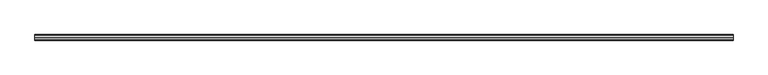
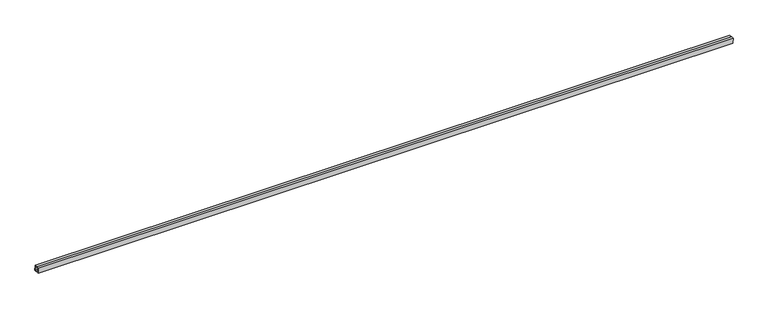
"""IFC4 building model written with IfcOpenShell, lengths in millimetres: proxy geometry, Inner panel:Inner panel:1:Inner panel:1 : Inner panel:Inner panel:300324:2:Inner panel:1:Inner panel:1 : Inner panel:Inner panel:300324:2 : Inner panel:Inner panel:1:Inner panel:1 : Inner panel:Inner panel:300324:300043:27 : Inner panel:Inner panel:1:Inner panel:1 : Inner panel:Inner panel:300324:2:Inner panel:1:Inner panel:1 : Inner panel:Inner panel:300324:2 : Inner panel:Inner panel:1:Inner panel:1 : Inner panel:Inner panel:300324:300043:308120."""

from ifc_helpers import new_model, si_unit, frame, origin, place, context, project, spatial, polyline, outline, extrude, source, transform, mapped, element, save


def generic_models_0cca4032(model_context):
    return source(origin(), model_context, "Body", "SweptSolid", [
        extrude(outline(polyline([(-567056.8153809, 8850.7720379), (-567038.5749577, 8851.5320556), (-567036.988834, 8813.4650855), (-567075.0558041, 8811.8789617), (-567076.6419278, 8849.9459318), (-567058.4015047, 8850.7059494), (-567058.3023719, 8848.3267638), (-567074.1636095, 8847.6658789), (-567072.7757512, 8814.3572801), (-567039.4671523, 8815.7451384), (-567040.8550106, 8849.0537372), (-567056.7162482, 8848.3928523), (-567056.8153809, 8850.7720379)])), frame((588245.3367242, 0.0, 0.0), z_axis=(1.0, 0.0, 0.0), x_axis=(0.0, 1.0, 0.0)), (0.0, 0.0, 1.0), 4876.8),
    ])


if __name__ == "__main__":
    model = new_model("IFC4")
    model_context = context("Model", 3, world=origin())
    ifc_project = project(units=[si_unit("LENGTHUNIT", "METRE", prefix="MILLI")], contexts=[model_context])
    site = spatial("IfcSite", under=ifc_project)
    building = spatial("IfcBuilding", under=site)
    placement = place(None, origin())
    generic_models_shape = generic_models_0cca4032(model_context)
    element("IfcBuildingElementProxy", 1, Name="Inner panel:Inner panel:1:Inner panel:1 : Inner panel:Inner panel:300324:2:Inner panel:1:Inner panel:1 : Inner panel:Inner panel:300324:2 : Inner panel:Inner panel:1:Inner panel:1 : Inner panel:Inner panel:300324:300043:27 : Inner panel:Inner panel:1:Inner panel:1 : Inner panel:Inner panel:300324:2:Inner panel:1:Inner panel:1 : Inner panel:Inner panel:300324:2 : Inner panel:Inner panel:1:Inner panel:1 : Inner panel:Inner panel:300324:300043:308120", ObjectType="Inner panel:Inner panel:1:Inner panel:1 : Inner panel:Inner panel:300324:2:Inner panel:1:Inner panel:1 : Inner panel:Inner panel:300324:2 : Inner panel:Inner panel:1:Inner panel:1 : Inner panel:Inner panel:300324:300043:27 : Inner panel:Inner panel:1:Inner panel:1 : Inner panel:Inner panel:300324:2:Inner panel:1:Inner panel:1 : Inner panel:Inner panel:300324:2 : Inner panel:Inner panel:1:Inner panel:1 : Inner panel:Inner panel:300324:300043:308120", at=placement, inside=building, context=model_context, shape_type="MappedRepresentation", body=[
        mapped(generic_models_shape, transform((0.0, 0.0, 0.0), x_axis=(1.0, 0.0, 0.0), y_axis=(0.0, 1.0, 0.0), z_axis=(0.0, 0.0, 1.0))),
    ])
    save(model, "model.ifc")

# Revit data of these elements
# Type "Inner panel:Inner panel:1:Inner panel:1 : Inner panel:Inner panel:300324:2:Inner panel:1:Inner panel:1 : Inner panel:Inner panel:300324:2 : Inner panel:Inner panel:1:Inner panel:1 : Inner panel:Inner panel:300324:300043:27 : Inner panel:Inner panel:1:Inner panel:1 : Inner panel:Inner panel:300324:2:Inner panel:1:Inner panel:1 : Inner panel:Inner panel:300324:2 : Inner panel:Inner panel:1:Inner panel:1 : Inner panel:Inner panel:300324:300043:308120"
#   NameOverride = "Inner panel:Inner panel:1:Inner panel:1 : Inner panel:Inner panel:300324:2:Inner panel:1:Inner panel:1 : Inner panel:Inner panel:300324:2 : Inner panel:Inner panel:1:Inner panel:1 : Inner panel:Inner panel:300324:300043:308120"
#   ObjectTypeOverride = "Inner panel:1:Inner panel:1 : Inner panel:Inner panel:300324:2 : Inner panel:Inner panel:1:Inner panel:1 : Inner panel:Inner panel:300324:300043"
#   Reference = "Inner panel"
#   Tag = "308120"
# Element 1 (IfcBuildingElementProxy, "Inner panel:Inner panel:1:Inner panel:1 : Inner panel:Inner panel:300324:2:Inner panel:1:Inner panel:1 : Inner panel:Inner panel:300324:2 : Inner panel:Inner panel:1:Inner panel:1 : Inner panel:Inner panel:300324:300043:27 : Inner panel:Inner panel:1:Inner panel:1 : Inner panel:Inner panel:300324:2:Inner panel:1:Inner panel:1 : Inner panel:Inner panel:300324:2 : Inner panel:Inner panel:1:Inner panel:1 : Inner panel:Inner panel:300324:300043:308120")
#   Materials on its faces: "1 1/2\" X 1 1/2\" SPLIT-SEAM SQUARE TUBING (~24\" CANTILEVER FROM C.L. OF GLULAM)"
# Materials
#   "1 1/2\" X 1 1/2\" SPLIT-SEAM SQUARE TUBING (~24\" CANTILEVER FROM C.L. OF GLULAM)": class "Unassigned", colour RGB 202 201 200, transparency 0, Cost = 0
